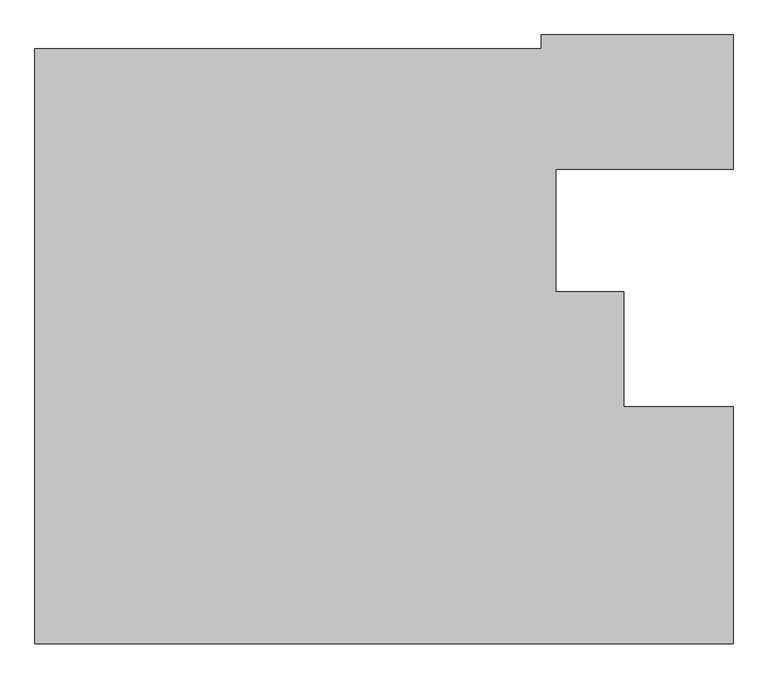
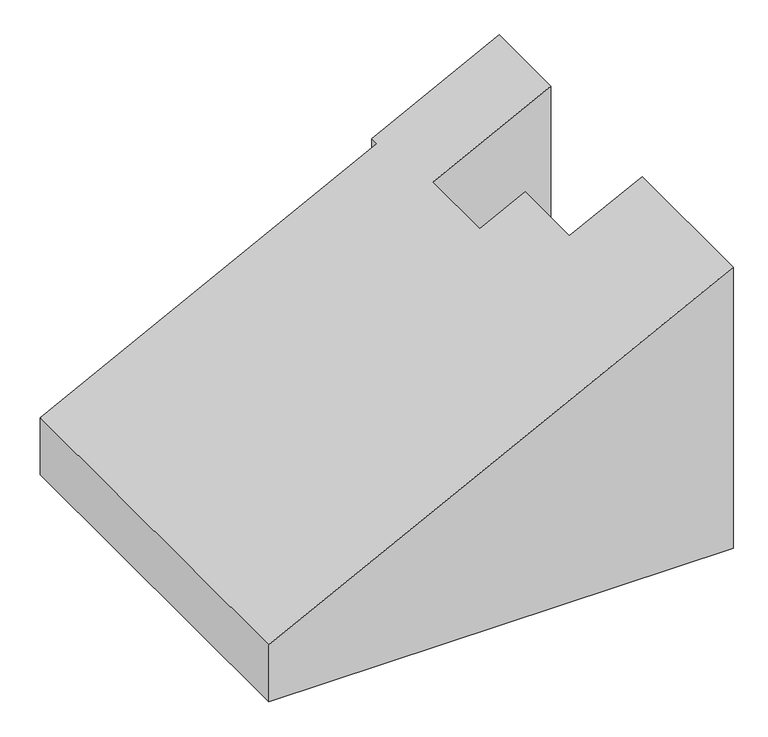
"""IFC4 building model written with IfcOpenShell, lengths in millimetres: proxy geometry, 0_3d_modell."""

from ifc_helpers import new_model, si_unit, origin, place, context, project, spatial, faceted_brep, source, transform, mapped, element, save


def generic_models_82b4d27e(model_context):
    return source(origin(), model_context, "Body", "Brep", [
        faceted_brep([(4750.0, 5582.8619019, 3273.5797924), (0.0, 5582.8619019, 853.3339073), (0.0, 0.0, 853.3339073), (6550.0, 0.0, 4190.7256015), (6550.0, 2223.2600653, 4190.7256015), (5525.0, 2223.2600653, 3668.4620158), (5525.0, 3302.8619019, 3668.4620158), (4885.0, 3302.8619019, 3342.3657281), (4885.0, 4452.8619019, 3342.3657281), (6550.0, 4452.8619019, 4190.7256015), (6550.0, 5712.8619019, 4190.7256015), (4750.0, 5712.8619019, 3273.5797924), (5525.0, 3302.8619019, 0.0), (4885.0, 3302.8619019, 0.0), (5525.0, 2223.2600653, 0.0), (6550.0, 2223.2600653, 0.0), (0.0, 0.0, 0.0), (6550.0, 0.0, 0.0), (0.0, 5582.8619019, 0.0), (4750.0, 5582.8619019, 0.0), (4750.0, 5712.8619019, 0.0), (6550.0, 5712.8619019, 0.0), (6550.0, 4452.8619019, 0.0), (4885.0, 4452.8619019, 0.0)], [[[0, 1, 2, 3, 4, 5, 6, 7, 8, 9, 10, 11]], [[7, 6, 12, 13]], [[6, 5, 14, 12]], [[5, 4, 15, 14]], [[3, 2, 16, 17]], [[2, 1, 18, 16]], [[1, 0, 19, 18]], [[0, 11, 20, 19]], [[11, 10, 21, 20]], [[22, 21, 10, 9]], [[9, 8, 23, 22]], [[8, 7, 13, 23]], [[17, 15, 4, 3]], [[16, 18, 19, 20, 21, 22, 23, 13, 12, 14, 15, 17]]]),
    ])


if __name__ == "__main__":
    model = new_model("IFC4")
    model_context = context("Model", 3, world=origin())
    ifc_project = project(units=[si_unit("LENGTHUNIT", "METRE", prefix="MILLI")], contexts=[model_context])
    site = spatial("IfcSite", under=ifc_project)
    building = spatial("IfcBuilding", under=site)
    placement = place(None, origin())
    generic_models_shape = generic_models_82b4d27e(model_context)
    element("IfcBuildingElementProxy", 1, Name="0_3d_modell", ObjectType="0_3d_modell", at=placement, inside=building, context=model_context, shape_type="MappedRepresentation", body=[
        mapped(generic_models_shape, transform((0.0, 0.0, 0.0), x_axis=(1.0, 0.0, 0.0), y_axis=(0.0, 1.0, 0.0), z_axis=(0.0, 0.0, 1.0))),
    ])
    save(model, "model.ifc")

# Revit data of these elements
# Element 1 (IfcBuildingElementProxy, "0_3d_modell")
#   Materials on its faces: "*1"
# Materials
#   "*1": class "Unassigned", colour RGB 175 175 175, transparency 0
